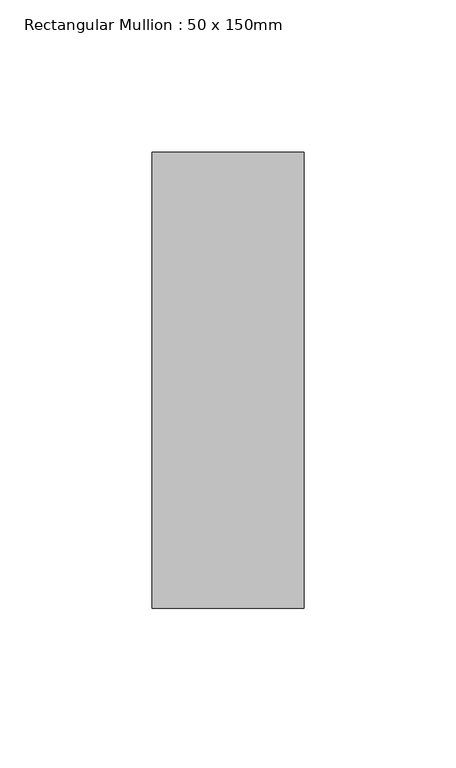
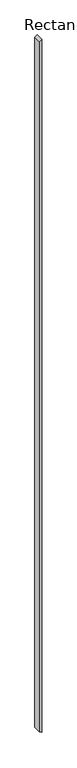
"""IFC4 building model written with IfcOpenShell, lengths in millimetres: member geometry, Rectangular Mullion : 50 x 150mm."""

import ifcopenshell
import ifcopenshell.guid

model = None  # the IFC model being written
_history = None  # IfcOwnerHistory: only IFC2X3 demands one
_inside = {}  # id of a spatial element -> (the spatial element, [elements in it])
_under = {}  # id of a project, library or spatial element -> (it, [spatial elements below it])
_declared = {}  # id of a project -> (the project, [libraries it declares])
_typed = {}  # id of a type object -> (the type object, [elements of that type])
_made_of = {}  # id of a material, layer set ... -> (it, [elements and type objects made of it])


def new_model(schema):
    """Start an empty IFC model of exactly this schema.

    Asked for "IFC4X3", IfcOpenShell would pick the latest addendum, in which some entities
    have other attributes; the version numbers below select the first issue.
    IFC2X3 requires an IfcOwnerHistory on every rooted entity: one is made here for all.
    """
    global model, _history
    if schema == "IFC4X3":
        model = ifcopenshell.file(schema_version=(4, 3, 0, 0))
    else:
        model = ifcopenshell.file(schema=schema)
    _inside.clear()
    _under.clear()
    _declared.clear()
    _typed.clear()
    _made_of.clear()
    _history = None
    if model.schema == "IFC2X3":
        org = make("IfcOrganization", Name="unknown")
        user = make(
            "IfcPersonAndOrganization",
            ThePerson=make("IfcPerson", FamilyName="unknown"),
            TheOrganization=org,
        )
        app = make(
            "IfcApplication",
            ApplicationDeveloper=org,
            Version="unknown",
            ApplicationFullName="unknown",
            ApplicationIdentifier="unknown",
        )
        _history = make(
            "IfcOwnerHistory",
            OwningUser=user,
            OwningApplication=app,
            ChangeAction="ADDED",
            CreationDate=0,
        )
    return model


def make(cls, **values):
    """One entity of the class cls with the attributes given. An attribute that is None is left unset."""
    return model.create_entity(
        cls, **{name: value for name, value in values.items() if value is not None}
    )


def rooted(cls, **values):
    """An entity with a GlobalId (a new one), such as an element, a storey or a relation."""
    return make(cls, GlobalId=ifcopenshell.guid.new(), OwnerHistory=_history, **values)


def si_unit(unit_type, name, prefix=None):
    """IfcSIUnit, for example si_unit("LENGTHUNIT", "METRE", prefix="MILLI")."""
    return make("IfcSIUnit", UnitType=unit_type, Prefix=prefix, Name=name)


def assignment(units):
    """IfcUnitAssignment: the units of a project."""
    return None if units is None else make("IfcUnitAssignment", Units=units)


def point(xyz):
    """IfcCartesianPoint."""
    return None if xyz is None else make("IfcCartesianPoint", Coordinates=xyz)


def direction(xyz):
    """IfcDirection."""
    return None if xyz is None else make("IfcDirection", DirectionRatios=xyz)


def frame(location, z_axis=None, x_axis=None):
    """IfcAxis2Placement3D, a coordinate frame: its origin and axes. An axis left out is left unset."""
    return make(
        "IfcAxis2Placement3D",
        Location=point(location),
        Axis=direction(z_axis),
        RefDirection=direction(x_axis),
    )


def origin():
    """The frame at (0, 0, 0) with its axes left unset."""
    return frame((0.0, 0.0, 0.0))


def place(relative_to, where):
    """IfcLocalPlacement: puts the frame where relative to a parent placement (None: the world)."""
    return make(
        "IfcLocalPlacement", PlacementRelTo=relative_to, RelativePlacement=where
    )


def context(
    kind, dimensions, precision=None, world=None, true_north=None, identifier=None
):
    """IfcGeometricRepresentationContext, for example the 3D "Model" context."""
    return make(
        "IfcGeometricRepresentationContext",
        ContextIdentifier=identifier,
        ContextType=kind,
        CoordinateSpaceDimension=dimensions,
        Precision=precision,
        WorldCoordinateSystem=world,
        TrueNorth=true_north,
    )


def project(units=None, contexts=None):
    """IfcProject with its units and contexts."""
    return rooted(
        "IfcProject",
        Name="project",
        RepresentationContexts=contexts,
        UnitsInContext=assignment(units),
    )


def spatial(cls, under=None, at=None, **own):
    """A site, building, storey or space (cls), placed at a placement, below another one or the project."""
    s = rooted(cls, ObjectPlacement=at, **own)
    if under is not None:
        _under.setdefault(under.id(), (under, []))[1].append(s)
    return s


def polyline(points):
    """IfcPolyline through the points."""
    return make("IfcPolyline", Points=[point(p) for p in points])


def outline(outer, holes=None, kind="AREA"):
    """IfcArbitraryClosedProfileDef: a profile drawn as a closed curve; with holes, ...WithVoids."""
    if holes is None:
        return make("IfcArbitraryClosedProfileDef", ProfileType=kind, OuterCurve=outer)
    return make(
        "IfcArbitraryProfileDefWithVoids",
        ProfileType=kind,
        OuterCurve=outer,
        InnerCurves=holes,
    )


def extrude(swept, where, along, depth):
    """IfcExtrudedAreaSolid: the profile swept, set in the frame where, extruded along a direction by depth."""
    return make(
        "IfcExtrudedAreaSolid",
        SweptArea=swept,
        Position=where,
        ExtrudedDirection=direction(along),
        Depth=depth,
    )


def shape(context_of_items, identifier, shape_type, items):
    """IfcShapeRepresentation: the items that make up one representation, for example the "Body"."""
    return make(
        "IfcShapeRepresentation",
        ContextOfItems=context_of_items,
        RepresentationIdentifier=identifier,
        RepresentationType=shape_type,
        Items=items,
    )


def source(mapping_origin, context_of_items, identifier, shape_type, items):
    """IfcRepresentationMap: a shape defined once, which mapped items show again and again."""
    return make(
        "IfcRepresentationMap",
        MappingOrigin=mapping_origin,
        MappedRepresentation=shape(context_of_items, identifier, shape_type, items),
    )


def transform(
    local_origin,
    x_axis=None,
    y_axis=None,
    z_axis=None,
    scale=None,
    scale2=None,
    scale3=None,
    uniform=True,
):
    """IfcCartesianTransformationOperator3D, or its non-uniform kind. x_axis, y_axis, z_axis: its Axis1, 2, 3."""
    if uniform:
        return make(
            "IfcCartesianTransformationOperator3D",
            Axis1=direction(x_axis),
            Axis2=direction(y_axis),
            LocalOrigin=point(local_origin),
            Scale=scale,
            Axis3=direction(z_axis),
        )
    return make(
        "IfcCartesianTransformationOperator3DnonUniform",
        Axis1=direction(x_axis),
        Axis2=direction(y_axis),
        LocalOrigin=point(local_origin),
        Scale=scale,
        Axis3=direction(z_axis),
        Scale2=scale2,
        Scale3=scale3,
    )


def mapped(mapping_source, mapping_target):
    """IfcMappedItem: shows the shape of a source again, moved by a transform."""
    return make(
        "IfcMappedItem", MappingSource=mapping_source, MappingTarget=mapping_target
    )


def made_of(thing, what):
    """Note that an element or type object is made of a material, layer set ...; save() writes the relation."""
    if what is not None:
        _made_of.setdefault(what.id(), (what, []))[1].append(thing)
    return thing


def element(
    cls,
    number,
    at=None,
    inside=None,
    cuts=None,
    type_object=None,
    material=None,
    context=None,
    identifier="Body",
    shape_type=None,
    held_by="IfcProductDefinitionShape",
    body=None,
    shapes=None,
    **own,
):
    """One element of the class cls, such as IfcWall. Its Tag is "e" and its number.

    at: its placement. inside: the storey or other place that contains it. cuts: it is an
    opening in that element (IfcRelVoidsElement). A single representation is given by context,
    identifier, shape_type and body (its items); several are given by shapes. held_by: the class
    of the entity that holds the representations. save() writes the other relations.
    """
    e = rooted(cls, Tag="e%d" % number, ObjectPlacement=at, **own)
    if body is not None:
        shapes = [shape(context, identifier, shape_type, body)]
    if shapes is not None:
        e.Representation = make(held_by, Representations=shapes)
    if inside is not None:
        _inside.setdefault(inside.id(), (inside, []))[1].append(e)
    if cuts is not None:
        rooted(
            "IfcRelVoidsElement", RelatingBuildingElement=cuts, RelatedOpeningElement=e
        )
    if type_object is not None:
        _typed.setdefault(type_object.id(), (type_object, []))[1].append(e)
    return made_of(e, material)


def aggregate(whole, parts):
    """IfcRelAggregates: a whole, such as a stair, and the parts it consists of."""
    return rooted("IfcRelAggregates", RelatingObject=whole, RelatedObjects=parts)


def save(model, path):
    """Write the relations noted so far, then the file.

    IfcRelAggregates (storeys below a building ...), IfcRelContainedInSpatialStructure (elements
    in a storey), IfcRelDefinesByType, IfcRelAssociatesMaterial and IfcRelDeclares: one each for
    every whole, place, type object, material and project.
    """
    for whole, parts in _under.values():
        aggregate(whole, parts)
    for where, things in _inside.values():
        rooted(
            "IfcRelContainedInSpatialStructure",
            RelatedElements=things,
            RelatingStructure=where,
        )
    for kind, things in _typed.values():
        rooted("IfcRelDefinesByType", RelatedObjects=things, RelatingType=kind)
    for what, things in _made_of.values():
        rooted("IfcRelAssociatesMaterial", RelatedObjects=things, RelatingMaterial=what)
    for by, libraries in _declared.values():
        rooted("IfcRelDeclares", RelatingContext=by, RelatedDefinitions=libraries)
    model.write(path)


def rectangular_mullion_50_x_150mm_72e471df(model_context):
    return source(origin(), model_context, "Body", "SweptSolid", [
        extrude(outline(polyline([(0.0, 0.0), (-34.9055374, -50.0), (-14669.1673585, -50.0), (-14698.4684276, 0.0), (0.0, 0.0)])), frame((0.0, -75.0, 0.0), z_axis=(0.0, 1.0, 0.0), x_axis=(0.0, 0.0, 1.0)), (0.0, 0.0, 1.0), 150.0),
    ])


if __name__ == "__main__":
    model = new_model("IFC4")
    model_context = context("Model", 3, world=origin())
    ifc_project = project(units=[si_unit("LENGTHUNIT", "METRE", prefix="MILLI")], contexts=[model_context])
    site = spatial("IfcSite", under=ifc_project)
    building = spatial("IfcBuilding", under=site)
    placement = place(None, origin())
    rectangular_mullion_50_x_150mm_shape = rectangular_mullion_50_x_150mm_72e471df(model_context)
    element("IfcMember", 1, ObjectType="Rectangular Mullion : 50 x 150mm", at=placement, inside=building, context=model_context, shape_type="MappedRepresentation", body=[
        mapped(rectangular_mullion_50_x_150mm_shape, transform((0.0, 0.0, 0.0), x_axis=(1.0, 0.0, 0.0), y_axis=(0.0, 1.0, 0.0), z_axis=(0.0, 0.0, 1.0))),
    ])
    save(model, "model.ifc")

# Revit data of these elements
# Type "Rectangular Mullion : 50 x 150mm"
#   built-in parameter 1007304 = 0.492126 (stored number, unit not read)
#   built-in parameter 1007301 = 0.082021 (stored number, unit not read)
#   built-in parameter 1007300 = 0.082021 (stored number, unit not read)
# Element 1 (IfcMember, "Rectangular Mullion : 50 x 150mm")
#   Materials on its faces: "Metal - Aluminium"
# Materials
#   "Metal - Aluminium": class "Metal", colour RGB 247 247 247, transparency 0
